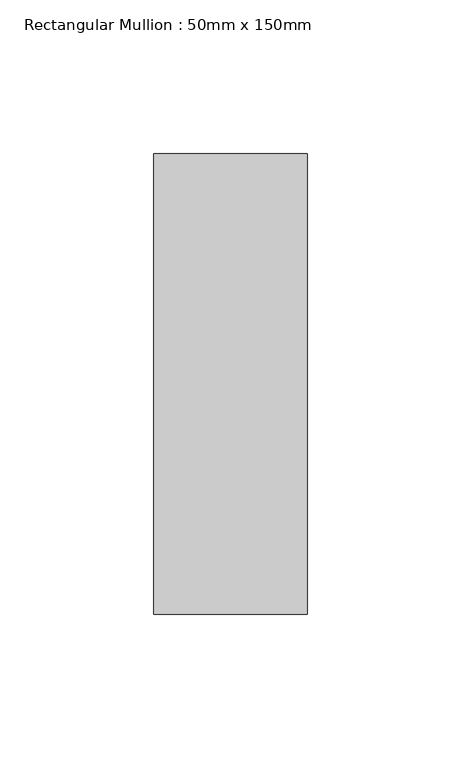
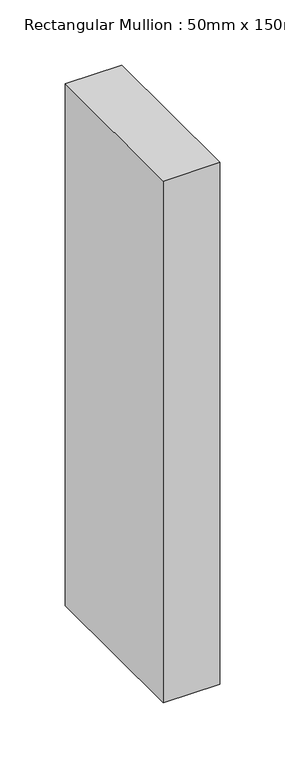
"""IFC4 building model written with IfcOpenShell, lengths in millimetres: member geometry, Rectangular Mullion : 50mm x 150mm."""

from ifc_helpers import new_model, si_unit, frame, origin, place, context, project, spatial, polyline, outline, extrude, source, transform, mapped, element, save


def rectangular_mullion_50mm_x_150mm_1a12905e(model_context):
    return source(origin(), model_context, "Body", "SweptSolid", [
        extrude(outline(polyline([(0.0, 75.0), (0.0, -75.0), (-50.0, -75.0), (-50.0, 75.0), (0.0, 75.0)])), frame((0.0, 0.0, -487.8787879), z_axis=(0.0, 0.0, 1.0), x_axis=(1.0, 0.0, 0.0)), (0.0, 0.0, 1.0), 487.8787879),
    ])


if __name__ == "__main__":
    model = new_model("IFC4")
    model_context = context("Model", 3, world=origin())
    ifc_project = project(units=[si_unit("LENGTHUNIT", "METRE", prefix="MILLI")], contexts=[model_context])
    site = spatial("IfcSite", under=ifc_project)
    building = spatial("IfcBuilding", under=site)
    placement = place(None, origin())
    rectangular_mullion_50mm_x_150mm_shape = rectangular_mullion_50mm_x_150mm_1a12905e(model_context)
    element("IfcMember", 1, ObjectType="Rectangular Mullion : 50mm x 150mm", at=placement, inside=building, context=model_context, shape_type="MappedRepresentation", body=[
        mapped(rectangular_mullion_50mm_x_150mm_shape, transform((0.0, 0.0, 0.0), x_axis=(1.0, 0.0, 0.0), y_axis=(0.0, 1.0, 0.0), z_axis=(0.0, 0.0, 1.0))),
    ])
    save(model, "model.ifc")

# Revit data of these elements
# Type "Rectangular Mullion : 50mm x 150mm"
#   built-in parameter 1007304 = 0.492126 (stored number, unit not read)
#   built-in parameter 1007301 = 0.082021 (stored number, unit not read)
#   built-in parameter 1007300 = 0.082021 (stored number, unit not read)
# Element 1 (IfcMember, "Rectangular Mullion : 50mm x 150mm")
#   Materials on its faces: "Aluminum"
# Materials
#   "Aluminum": class "Metal", colour RGB 244 244 244, transparency 0, Description = "Aluminum 6061", Cost = 0
